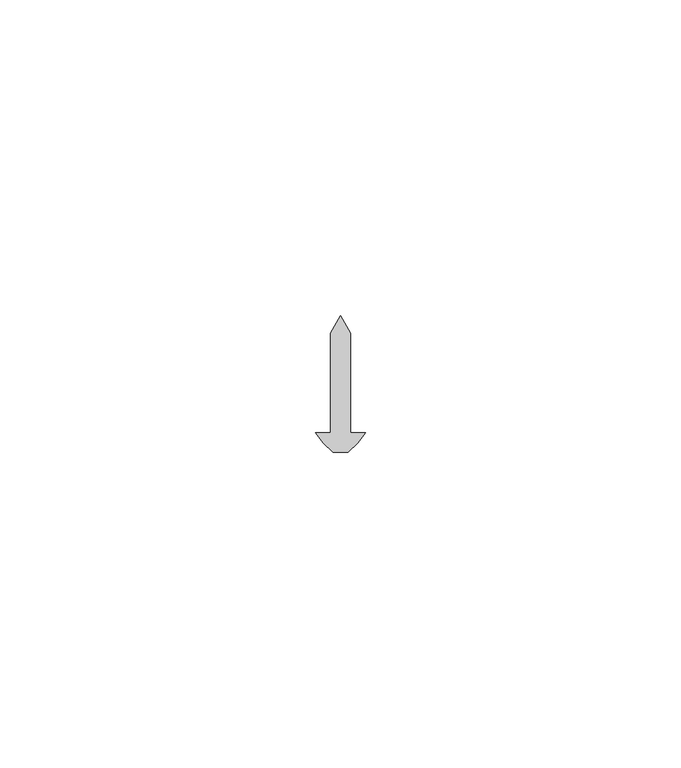
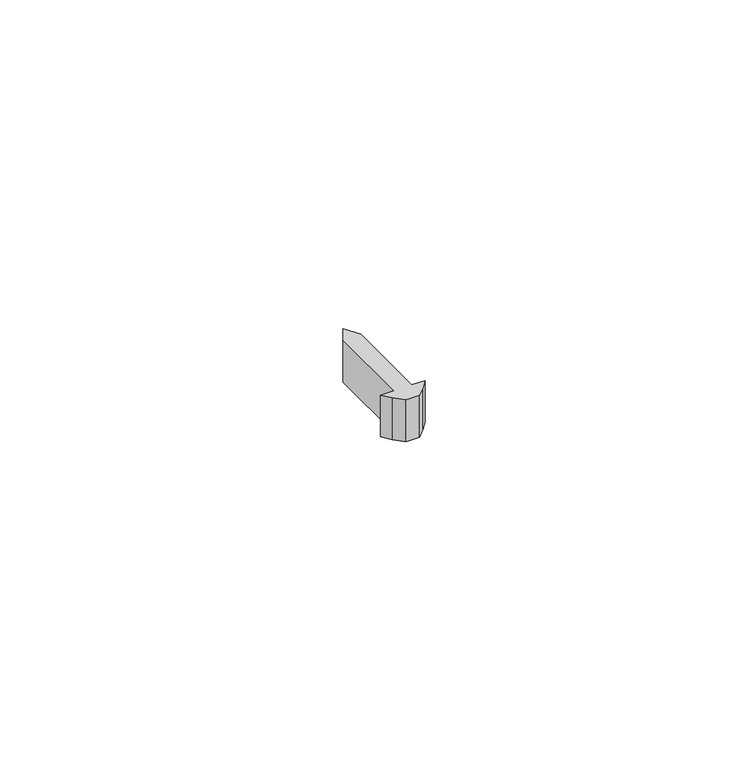
"""IFC4 building model written with IfcOpenShell, lengths in millimetres: proxy geometry, Generic Models 7:Generic Models 1:3:Generic Models 1:3 : Generic Models 7:Generic Models 1:305549:3:Generic Models 1:3:Generic Models 1:3 : Generic Models 7:Generic Models 1:305549:3 : Generic Models 7:Generic Models 1:3:Generic Models 1:3 : Generic Models 7:Generic Models 1:305549:301244:44 : Generic Models 7:Generic Models 1:3:Generic Models 1:3 : Generic Models 7:Generic Models 1:305549:3:Generic Models 1:3:Generic Models 1:3 : Generic Models 7:Generic Models 1:305549:3 : Generic Models 7:Generic Models 1:3:Generic Models 1:3 : Generic Models 7:Generic Models 1:305549:301244:308848."""

import ifcopenshell
import ifcopenshell.guid

model = None  # the IFC model being written
_history = None  # IfcOwnerHistory: only IFC2X3 demands one
_inside = {}  # id of a spatial element -> (the spatial element, [elements in it])
_under = {}  # id of a project, library or spatial element -> (it, [spatial elements below it])
_declared = {}  # id of a project -> (the project, [libraries it declares])
_typed = {}  # id of a type object -> (the type object, [elements of that type])
_made_of = {}  # id of a material, layer set ... -> (it, [elements and type objects made of it])


def new_model(schema):
    """Start an empty IFC model of exactly this schema.

    Asked for "IFC4X3", IfcOpenShell would pick the latest addendum, in which some entities
    have other attributes; the version numbers below select the first issue.
    IFC2X3 requires an IfcOwnerHistory on every rooted entity: one is made here for all.
    """
    global model, _history
    if schema == "IFC4X3":
        model = ifcopenshell.file(schema_version=(4, 3, 0, 0))
    else:
        model = ifcopenshell.file(schema=schema)
    _inside.clear()
    _under.clear()
    _declared.clear()
    _typed.clear()
    _made_of.clear()
    _history = None
    if model.schema == "IFC2X3":
        org = make("IfcOrganization", Name="unknown")
        user = make(
            "IfcPersonAndOrganization",
            ThePerson=make("IfcPerson", FamilyName="unknown"),
            TheOrganization=org,
        )
        app = make(
            "IfcApplication",
            ApplicationDeveloper=org,
            Version="unknown",
            ApplicationFullName="unknown",
            ApplicationIdentifier="unknown",
        )
        _history = make(
            "IfcOwnerHistory",
            OwningUser=user,
            OwningApplication=app,
            ChangeAction="ADDED",
            CreationDate=0,
        )
    return model


def make(cls, **values):
    """One entity of the class cls with the attributes given. An attribute that is None is left unset."""
    return model.create_entity(
        cls, **{name: value for name, value in values.items() if value is not None}
    )


def rooted(cls, **values):
    """An entity with a GlobalId (a new one), such as an element, a storey or a relation."""
    return make(cls, GlobalId=ifcopenshell.guid.new(), OwnerHistory=_history, **values)


def si_unit(unit_type, name, prefix=None):
    """IfcSIUnit, for example si_unit("LENGTHUNIT", "METRE", prefix="MILLI")."""
    return make("IfcSIUnit", UnitType=unit_type, Prefix=prefix, Name=name)


def assignment(units):
    """IfcUnitAssignment: the units of a project."""
    return None if units is None else make("IfcUnitAssignment", Units=units)


def point(xyz):
    """IfcCartesianPoint."""
    return None if xyz is None else make("IfcCartesianPoint", Coordinates=xyz)


def direction(xyz):
    """IfcDirection."""
    return None if xyz is None else make("IfcDirection", DirectionRatios=xyz)


def frame(location, z_axis=None, x_axis=None):
    """IfcAxis2Placement3D, a coordinate frame: its origin and axes. An axis left out is left unset."""
    return make(
        "IfcAxis2Placement3D",
        Location=point(location),
        Axis=direction(z_axis),
        RefDirection=direction(x_axis),
    )


def origin():
    """The frame at (0, 0, 0) with its axes left unset."""
    return frame((0.0, 0.0, 0.0))


def place(relative_to, where):
    """IfcLocalPlacement: puts the frame where relative to a parent placement (None: the world)."""
    return make(
        "IfcLocalPlacement", PlacementRelTo=relative_to, RelativePlacement=where
    )


def context(
    kind, dimensions, precision=None, world=None, true_north=None, identifier=None
):
    """IfcGeometricRepresentationContext, for example the 3D "Model" context."""
    return make(
        "IfcGeometricRepresentationContext",
        ContextIdentifier=identifier,
        ContextType=kind,
        CoordinateSpaceDimension=dimensions,
        Precision=precision,
        WorldCoordinateSystem=world,
        TrueNorth=true_north,
    )


def project(units=None, contexts=None):
    """IfcProject with its units and contexts."""
    return rooted(
        "IfcProject",
        Name="project",
        RepresentationContexts=contexts,
        UnitsInContext=assignment(units),
    )


def spatial(cls, under=None, at=None, **own):
    """A site, building, storey or space (cls), placed at a placement, below another one or the project."""
    s = rooted(cls, ObjectPlacement=at, **own)
    if under is not None:
        _under.setdefault(under.id(), (under, []))[1].append(s)
    return s


def polyline(points):
    """IfcPolyline through the points."""
    return make("IfcPolyline", Points=[point(p) for p in points])


def outline(outer, holes=None, kind="AREA"):
    """IfcArbitraryClosedProfileDef: a profile drawn as a closed curve; with holes, ...WithVoids."""
    if holes is None:
        return make("IfcArbitraryClosedProfileDef", ProfileType=kind, OuterCurve=outer)
    return make(
        "IfcArbitraryProfileDefWithVoids",
        ProfileType=kind,
        OuterCurve=outer,
        InnerCurves=holes,
    )


def extrude(swept, where, along, depth):
    """IfcExtrudedAreaSolid: the profile swept, set in the frame where, extruded along a direction by depth."""
    return make(
        "IfcExtrudedAreaSolid",
        SweptArea=swept,
        Position=where,
        ExtrudedDirection=direction(along),
        Depth=depth,
    )


def shape(context_of_items, identifier, shape_type, items):
    """IfcShapeRepresentation: the items that make up one representation, for example the "Body"."""
    return make(
        "IfcShapeRepresentation",
        ContextOfItems=context_of_items,
        RepresentationIdentifier=identifier,
        RepresentationType=shape_type,
        Items=items,
    )


def source(mapping_origin, context_of_items, identifier, shape_type, items):
    """IfcRepresentationMap: a shape defined once, which mapped items show again and again."""
    return make(
        "IfcRepresentationMap",
        MappingOrigin=mapping_origin,
        MappedRepresentation=shape(context_of_items, identifier, shape_type, items),
    )


def transform(
    local_origin,
    x_axis=None,
    y_axis=None,
    z_axis=None,
    scale=None,
    scale2=None,
    scale3=None,
    uniform=True,
):
    """IfcCartesianTransformationOperator3D, or its non-uniform kind. x_axis, y_axis, z_axis: its Axis1, 2, 3."""
    if uniform:
        return make(
            "IfcCartesianTransformationOperator3D",
            Axis1=direction(x_axis),
            Axis2=direction(y_axis),
            LocalOrigin=point(local_origin),
            Scale=scale,
            Axis3=direction(z_axis),
        )
    return make(
        "IfcCartesianTransformationOperator3DnonUniform",
        Axis1=direction(x_axis),
        Axis2=direction(y_axis),
        LocalOrigin=point(local_origin),
        Scale=scale,
        Axis3=direction(z_axis),
        Scale2=scale2,
        Scale3=scale3,
    )


def mapped(mapping_source, mapping_target):
    """IfcMappedItem: shows the shape of a source again, moved by a transform."""
    return make(
        "IfcMappedItem", MappingSource=mapping_source, MappingTarget=mapping_target
    )


def made_of(thing, what):
    """Note that an element or type object is made of a material, layer set ...; save() writes the relation."""
    if what is not None:
        _made_of.setdefault(what.id(), (what, []))[1].append(thing)
    return thing


def element(
    cls,
    number,
    at=None,
    inside=None,
    cuts=None,
    type_object=None,
    material=None,
    context=None,
    identifier="Body",
    shape_type=None,
    held_by="IfcProductDefinitionShape",
    body=None,
    shapes=None,
    **own,
):
    """One element of the class cls, such as IfcWall. Its Tag is "e" and its number.

    at: its placement. inside: the storey or other place that contains it. cuts: it is an
    opening in that element (IfcRelVoidsElement). A single representation is given by context,
    identifier, shape_type and body (its items); several are given by shapes. held_by: the class
    of the entity that holds the representations. save() writes the other relations.
    """
    e = rooted(cls, Tag="e%d" % number, ObjectPlacement=at, **own)
    if body is not None:
        shapes = [shape(context, identifier, shape_type, body)]
    if shapes is not None:
        e.Representation = make(held_by, Representations=shapes)
    if inside is not None:
        _inside.setdefault(inside.id(), (inside, []))[1].append(e)
    if cuts is not None:
        rooted(
            "IfcRelVoidsElement", RelatingBuildingElement=cuts, RelatedOpeningElement=e
        )
    if type_object is not None:
        _typed.setdefault(type_object.id(), (type_object, []))[1].append(e)
    return made_of(e, material)


def aggregate(whole, parts):
    """IfcRelAggregates: a whole, such as a stair, and the parts it consists of."""
    return rooted("IfcRelAggregates", RelatingObject=whole, RelatedObjects=parts)


def save(model, path):
    """Write the relations noted so far, then the file.

    IfcRelAggregates (storeys below a building ...), IfcRelContainedInSpatialStructure (elements
    in a storey), IfcRelDefinesByType, IfcRelAssociatesMaterial and IfcRelDeclares: one each for
    every whole, place, type object, material and project.
    """
    for whole, parts in _under.values():
        aggregate(whole, parts)
    for where, things in _inside.values():
        rooted(
            "IfcRelContainedInSpatialStructure",
            RelatedElements=things,
            RelatingStructure=where,
        )
    for kind, things in _typed.values():
        rooted("IfcRelDefinesByType", RelatedObjects=things, RelatingType=kind)
    for what, things in _made_of.values():
        rooted("IfcRelAssociatesMaterial", RelatedObjects=things, RelatingMaterial=what)
    for by, libraries in _declared.values():
        rooted("IfcRelDeclares", RelatingContext=by, RelatedDefinitions=libraries)
    model.write(path)


def generic_models_02dd9ac8(model_context):
    return source(origin(), model_context, "Body", "SweptSolid", [
        extrude(outline(polyline([(560618.0742239, -579084.8288841), (560620.4554739, -579084.8288841), (560619.2372784, -579086.3559421), (560617.6853882, -579087.9078323), (560615.2880597, -579087.9078323), (560613.7361695, -579086.3559421), (560612.5179739, -579084.8288841), (560614.8992239, -579084.8288841), (560614.8992239, -579069.0196286), (560616.4867239, -579066.2699979), (560618.0742239, -579069.0196286), (560618.0742239, -579084.8288841)])), frame((0.0, 0.0, 4907.75625), z_axis=(0.0, 0.0, 1.0), x_axis=(1.0, 0.0, 0.0)), (0.0, 0.0, 1.0), 7.9375),
    ])


if __name__ == "__main__":
    model = new_model("IFC4")
    model_context = context("Model", 3, world=origin())
    ifc_project = project(units=[si_unit("LENGTHUNIT", "METRE", prefix="MILLI")], contexts=[model_context])
    site = spatial("IfcSite", under=ifc_project)
    building = spatial("IfcBuilding", under=site)
    placement = place(None, origin())
    generic_models_shape = generic_models_02dd9ac8(model_context)
    element("IfcBuildingElementProxy", 1, Name="Generic Models 7:Generic Models 1:3:Generic Models 1:3 : Generic Models 7:Generic Models 1:305549:3:Generic Models 1:3:Generic Models 1:3 : Generic Models 7:Generic Models 1:305549:3 : Generic Models 7:Generic Models 1:3:Generic Models 1:3 : Generic Models 7:Generic Models 1:305549:301244:44 : Generic Models 7:Generic Models 1:3:Generic Models 1:3 : Generic Models 7:Generic Models 1:305549:3:Generic Models 1:3:Generic Models 1:3 : Generic Models 7:Generic Models 1:305549:3 : Generic Models 7:Generic Models 1:3:Generic Models 1:3 : Generic Models 7:Generic Models 1:305549:301244:308848", ObjectType="Generic Models 7:Generic Models 1:3:Generic Models 1:3 : Generic Models 7:Generic Models 1:305549:3:Generic Models 1:3:Generic Models 1:3 : Generic Models 7:Generic Models 1:305549:3 : Generic Models 7:Generic Models 1:3:Generic Models 1:3 : Generic Models 7:Generic Models 1:305549:301244:44 : Generic Models 7:Generic Models 1:3:Generic Models 1:3 : Generic Models 7:Generic Models 1:305549:3:Generic Models 1:3:Generic Models 1:3 : Generic Models 7:Generic Models 1:305549:3 : Generic Models 7:Generic Models 1:3:Generic Models 1:3 : Generic Models 7:Generic Models 1:305549:301244:308848", at=placement, inside=building, context=model_context, shape_type="MappedRepresentation", body=[
        mapped(generic_models_shape, transform((0.0, 0.0, 0.0), x_axis=(1.0, 0.0, 0.0), y_axis=(0.0, 1.0, 0.0), z_axis=(0.0, 0.0, 1.0))),
    ])
    save(model, "model.ifc")

# Revit data of these elements
# Type "Generic Models 7:Generic Models 1:3:Generic Models 1:3 : Generic Models 7:Generic Models 1:305549:3:Generic Models 1:3:Generic Models 1:3 : Generic Models 7:Generic Models 1:305549:3 : Generic Models 7:Generic Models 1:3:Generic Models 1:3 : Generic Models 7:Generic Models 1:305549:301244:44 : Generic Models 7:Generic Models 1:3:Generic Models 1:3 : Generic Models 7:Generic Models 1:305549:3:Generic Models 1:3:Generic Models 1:3 : Generic Models 7:Generic Models 1:305549:3 : Generic Models 7:Generic Models 1:3:Generic Models 1:3 : Generic Models 7:Generic Models 1:305549:301244:308848"
#   NameOverride = "Generic Models 7:Generic Models 1:3:Generic Models 1:3 : Generic Models 7:Generic Models 1:305549:3:Generic Models 1:3:Generic Models 1:3 : Generic Models 7:Generic Models 1:305549:3 : Generic Models 7:Generic Models 1:3:Generic Models 1:3 : Generic Models 7:Generic Models 1:305549:301244:308848"
#   ObjectTypeOverride = "Generic Models 1:3:Generic Models 1:3 : Generic Models 7:Generic Models 1:305549:3 : Generic Models 7:Generic Models 1:3:Generic Models 1:3 : Generic Models 7:Generic Models 1:305549:301244"
#   Reference = "Generic Models 1"
#   Tag = "308848"
# Element 1 (IfcBuildingElementProxy, "Generic Models 7:Generic Models 1:3:Generic Models 1:3 : Generic Models 7:Generic Models 1:305549:3:Generic Models 1:3:Generic Models 1:3 : Generic Models 7:Generic Models 1:305549:3 : Generic Models 7:Generic Models 1:3:Generic Models 1:3 : Generic Models 7:Generic Models 1:305549:301244:44 : Generic Models 7:Generic Models 1:3:Generic Models 1:3 : Generic Models 7:Generic Models 1:305549:3:Generic Models 1:3:Generic Models 1:3 : Generic Models 7:Generic Models 1:305549:3 : Generic Models 7:Generic Models 1:3:Generic Models 1:3 : Generic Models 7:Generic Models 1:305549:301244:308848")
#   Materials on its faces: "FASTENERS (T.B.D)"
# Materials
#   "FASTENERS (T.B.D)": class "Generic", colour RGB 120 120 120, transparency 0, Cost = 0
